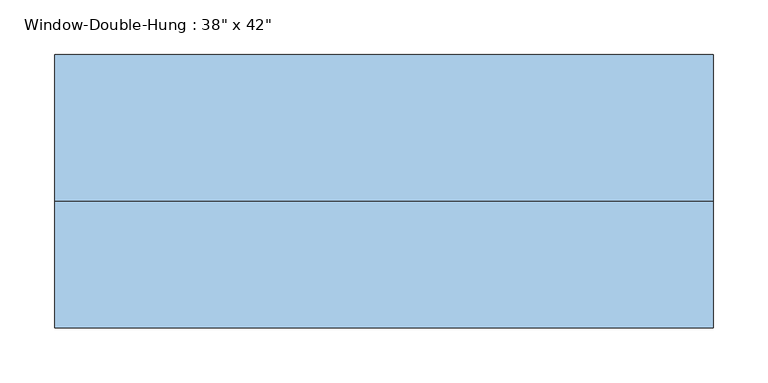
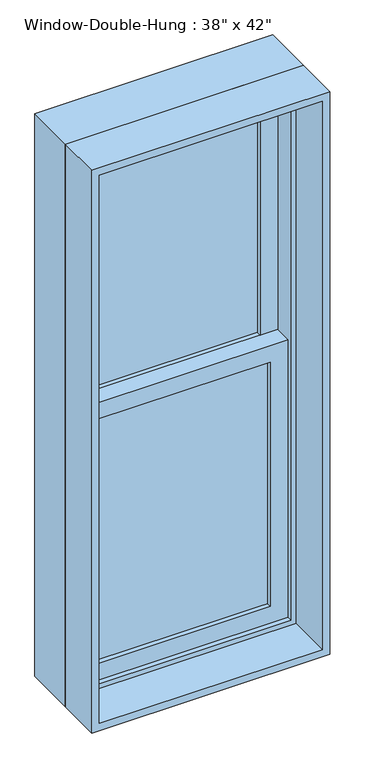
"""IFC4 building model written with IfcOpenShell, lengths in millimetres: window geometry."""

from ifc_helpers import new_model, si_unit, frame, origin, place, context, project, spatial, polyline, outline, extrude, source, transform, mapped, element, save


def window_22e1c68e(model_context):
    return source(origin(), model_context, "Body", "SweptSolid", [
        extrude(outline(polyline([(223.8, 45.15), (223.8, 38.8), (-223.8, 38.8), (-223.8, 45.15), (223.8, 45.15)])), frame((0.0, 0.0, 990.6), z_axis=(0.0, 0.0, 1.0), x_axis=(1.0, 0.0, 0.0)), (0.0, 0.0, 1.0), 651.575),
        extrude(outline(polyline([(-223.8, 32.45), (223.8, 32.45), (223.8, 26.1), (-223.8, 26.1), (-223.8, 32.45)])), frame((0.0, 0.0, 990.6), z_axis=(0.0, 0.0, 1.0), x_axis=(1.0, 0.0, 0.0)), (0.0, 0.0, 1.0), 651.575),
        extrude(outline(polyline([(223.8, 89.6), (223.8, 83.25), (-223.8, 83.25), (-223.8, 89.6), (223.8, 89.6)])), frame((0.0, 0.0, 1686.625), z_axis=(0.0, 0.0, 1.0), x_axis=(1.0, 0.0, 0.0)), (0.0, 0.0, 1.0), 651.575),
        extrude(outline(polyline([(-223.8, 76.9), (223.8, 76.9), (223.8, 70.55), (-223.8, 70.55), (-223.8, 76.9)])), frame((0.0, 0.0, 1686.625), z_axis=(0.0, 0.0, 1.0), x_axis=(1.0, 0.0, 0.0)), (0.0, 0.0, 1.0), 651.575),
        extrude(outline(polyline([(1686.625, -268.25), (946.15, -268.25), (946.15, 268.25), (1686.625, 268.25), (1686.625, -268.25)]), holes=[polyline([(1642.175, 223.8), (990.6, 223.8), (990.6, -223.8), (1642.175, -223.8), (1642.175, 223.8)])]), frame((0.0, 13.4, 0.0), z_axis=(0.0, 1.0, 0.0), x_axis=(0.0, 0.0, 1.0)), (0.0, 0.0, 1.0), 44.45),
        extrude(outline(polyline([(2382.65, -268.25), (1642.175, -268.25), (1642.175, 268.25), (2382.65, 268.25), (2382.65, -268.25)]), holes=[polyline([(2338.2, 223.8), (1686.625, 223.8), (1686.625, -223.8), (2338.2, -223.8), (2338.2, 223.8)])]), frame((0.0, 57.85, 0.0), z_axis=(0.0, 1.0, 0.0), x_axis=(0.0, 0.0, 1.0)), (0.0, 0.0, 1.0), 44.45),
        extrude(outline(polyline([(2414.4, -300.0), (914.4, -300.0), (914.4, 300.0), (2414.4, 300.0), (2414.4, -300.0)]), holes=[polyline([(2382.65, 268.25), (946.15, 268.25), (946.15, -268.25), (2382.65, -268.25), (2382.65, 268.25)])]), frame((0.0, 0.7, 0.0), z_axis=(0.0, 1.0, 0.0), x_axis=(0.0, 0.0, 1.0)), (0.0, 0.0, 1.0), 133.35),
        extrude(outline(polyline([(2414.4, 300.0), (2414.4, -300.0), (914.4, -300.0), (914.4, 300.0), (2414.4, 300.0)]), holes=[polyline([(2395.35, 280.95), (933.45, 280.95), (933.45, -280.95), (2395.35, -280.95), (2395.35, 280.95)])]), frame((0.0, -115.0, 0.0), z_axis=(0.0, 1.0, 0.0), x_axis=(0.0, 0.0, 1.0)), (0.0, 0.0, 1.0), 115.7),
    ])


if __name__ == "__main__":
    model = new_model("IFC4")
    model_context = context("Model", 3, world=origin())
    ifc_project = project(units=[si_unit("LENGTHUNIT", "METRE", prefix="MILLI")], contexts=[model_context])
    site = spatial("IfcSite", under=ifc_project)
    building = spatial("IfcBuilding", under=site)
    placement = place(None, origin())
    window_shape = window_22e1c68e(model_context)
    element("IfcWindow", 1, ObjectType="Window-Double-Hung : 38\" x 42\"", at=placement, inside=building, context=model_context, shape_type="MappedRepresentation", body=[
        mapped(window_shape, transform((0.0, 0.0, 0.0), x_axis=(1.0, 0.0, 0.0), y_axis=(0.0, 1.0, 0.0), z_axis=(0.0, 0.0, 1.0))),
    ])
    save(model, "model.ifc")

# Revit data of these elements
# Type "Window-Double-Hung : 38\" x 42\""
#   Type Mark = "38"
#   Fire Rating = "0.5h"
#   Construction Type Id = "DG-DR"
#   Assembly Code = "B2020100"
#   Analytic Construction = "Double glazing - domestic"
#   Wall Thickness [instance default] = 15.24 cm
#   Window Inset [instance default] = 0 cm
#   Visual Light Transmittance = 0.81
#   Thermal Resistance (R) = 0.319569 (m²·K)/W
#   Solar Heat Gain Coefficient = 0.76
#   Muntin Width = 44.76 cm
#   Muntin Height = 65.1575 cm
#   Interior Wall Closure [instance default] = 3.81 cm
#   Rough Width = 61.27 cm
#   Rough Height = 151.27 cm
#   Frame Extension [instance default] = 3.175 cm
#   Exterior Wall Closure [instance default] = 1.27 cm
#   Extension Jamb [instance default] = 3.81 cm
#   Heat Transfer Coefficient (U) = 3.12929 W/(m²·K)
#   Height = 150 cm
#   Width = 60 cm
#   Top Muntin Visibility = yes
#   Indicator Visibility [instance default] = yes
#   Extension Jamb Visibility [instance default] = yes
#   Interior Trim Visibility [instance default] = yes
#   Exterior Trim Visibility [instance default] = yes
#   Bottom Muntin Visibility = yes
#   Muntin Pattern = Muntin Pattern_2x2 : Muntin Pattern_2x2
#   Interior Trim Material = Wood - Stained
#   Interior Trim = Trim-Window-Interior-Flat : Picture Frame
#   Exterior Trim Material = Clad - White
#   Exterior Trim = Trim-Window-Exterior-Flat : with Sill
#   Glass Panel Material = Glass
#   Exterior Frame Material = Clad - White
#   Interior Frame Material = Wood - Stained
#   Wall Closure = (empty or 0)
# Element 1 (IfcWindow, "Window-Double-Hung : 38\" x 42\"")
#   Wall Thickness = 23 cm
#   Extension Jamb = 11.57 cm
#   Materials on its faces: "Wood - Stained", "Glass", "Clad - White"
# Materials
#   "Wood - Stained": class "Wood", colour RGB 224 178 126, transparency 0, Cost = 0
#   "Clad - White": class "Wood", colour RGB 242 242 238, transparency 0, Cost = 0
#   "Glass": class "Glass", colour RGB 0 128 192, transparency 0.9, Description = "Soda Lime Glass", Cost = 0
